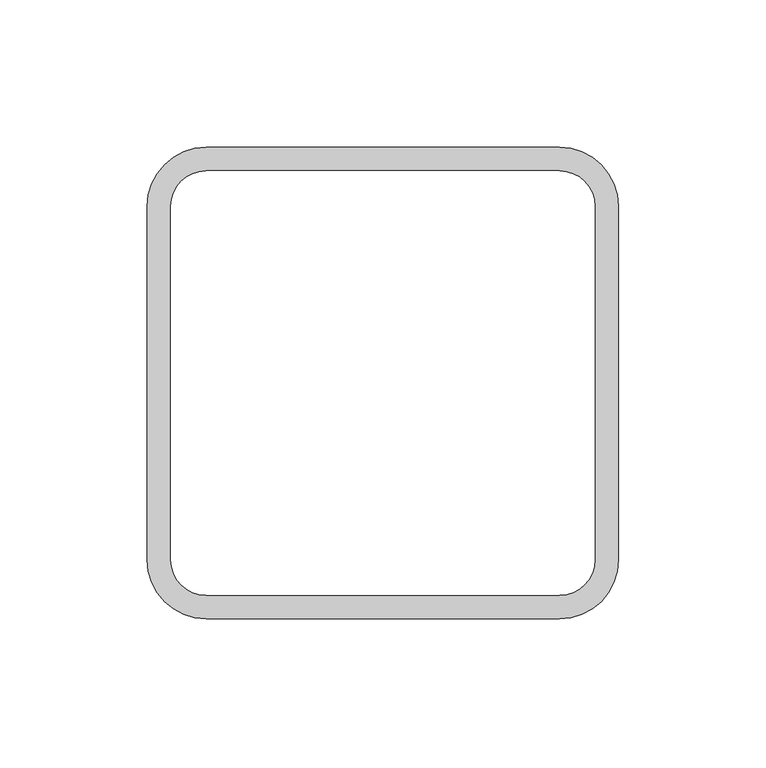
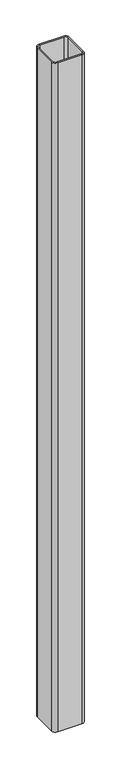
"""IFC4 building model written with IfcOpenShell, lengths in millimetres: column geometry, NLRS_28_SCO_TLB_stalen kolom buisprofiel koudgevormd vierkant-BCPG-MMBS-SRP_gen_rsf : stalen kolom buisprofiel koudgevormd vierkant RHSC_gen__160x160x8."""

from ifc_helpers import new_model, si_unit, point, frame, frame_2d, origin, place, context, project, spatial, polyline, circle_curve, trimmed, segment, composite_curve, outline, extrude, source, transform, mapped, element, save


def column_d8346d76(model_context):
    return source(origin(), model_context, "Body", "SweptSolid", [
        extrude(outline(composite_curve([segment(trimmed(circle_curve(frame_2d((60.0, 60.0)), 20.0), [point((60.0, 80.0))], [point((80.0, 60.0))], False, "CARTESIAN"), True, "CONTINUOUS"), segment(polyline([(80.0, 60.0), (80.0, -60.0)]), True, "CONTINUOUS"), segment(trimmed(circle_curve(frame_2d((60.0, -60.0)), 20.0), [point((80.0, -60.0))], [point((60.0, -80.0))], False, "CARTESIAN"), True, "CONTINUOUS"), segment(polyline([(60.0, -80.0), (-60.0, -80.0)]), True, "CONTINUOUS"), segment(trimmed(circle_curve(frame_2d((-60.0, -60.0)), 20.0), [point((-60.0, -80.0))], [point((-80.0, -60.0))], False, "CARTESIAN"), True, "CONTINUOUS"), segment(polyline([(-80.0, -60.0), (-80.0, 60.0)]), True, "CONTINUOUS"), segment(trimmed(circle_curve(frame_2d((-60.0, 60.0)), 20.0), [point((-80.0, 60.0))], [point((-60.0, 80.0))], False, "CARTESIAN"), True, "CONTINUOUS"), segment(polyline([(-60.0, 80.0), (60.0, 80.0)]), True, "CONTINUOUS")], self_intersect=False), holes=[composite_curve([segment(polyline([(60.0, 72.0), (-60.0, 72.0)]), True, "CONTINUOUS"), segment(trimmed(circle_curve(frame_2d((-60.0, 60.0)), 12.0), [point((-60.0, 72.0))], [point((-72.0, 60.0))], True, "CARTESIAN"), True, "CONTINUOUS"), segment(polyline([(-72.0, 60.0), (-72.0, -60.0)]), True, "CONTINUOUS"), segment(trimmed(circle_curve(frame_2d((-60.0, -60.0)), 12.0), [point((-72.0, -60.0))], [point((-60.0, -72.0))], True, "CARTESIAN"), True, "CONTINUOUS"), segment(polyline([(-60.0, -72.0), (60.0, -72.0)]), True, "CONTINUOUS"), segment(trimmed(circle_curve(frame_2d((60.0, -60.0)), 12.0), [point((60.0, -72.0))], [point((72.0, -60.0))], True, "CARTESIAN"), True, "CONTINUOUS"), segment(polyline([(72.0, -60.0), (72.0, 60.0)]), True, "CONTINUOUS"), segment(trimmed(circle_curve(frame_2d((60.0, 60.0)), 12.0), [point((72.0, 60.0))], [point((60.0, 72.0))], True, "CARTESIAN"), True, "CONTINUOUS")], self_intersect=False)]), frame((0.0, 0.0, -40.0), z_axis=(0.0, 0.0, 1.0), x_axis=(1.0, 0.0, 0.0)), (0.0, 0.0, 1.0), 3510.0),
    ])


if __name__ == "__main__":
    model = new_model("IFC4")
    model_context = context("Model", 3, world=origin())
    ifc_project = project(units=[si_unit("LENGTHUNIT", "METRE", prefix="MILLI")], contexts=[model_context])
    site = spatial("IfcSite", under=ifc_project)
    building = spatial("IfcBuilding", under=site)
    placement = place(None, origin())
    column_shape = column_d8346d76(model_context)
    element("IfcColumn", 1, ObjectType="NLRS_28_SCO_TLB_stalen kolom buisprofiel koudgevormd vierkant-BCPG-MMBS-SRP_gen_rsf : stalen kolom buisprofiel koudgevormd vierkant RHSC_gen__160x160x8", at=placement, inside=building, context=model_context, shape_type="MappedRepresentation", body=[
        mapped(column_shape, transform((0.0, 0.0, 0.0), x_axis=(1.0, 0.0, 0.0), y_axis=(0.0, 1.0, 0.0), z_axis=(0.0, 0.0, 1.0))),
    ])
    save(model, "model.ifc")

# Revit data of these elements
# Type "NLRS_28_SCO_TLB_stalen kolom buisprofiel koudgevormd vierkant-BCPG-MMBS-SRP_gen_rsf : stalen kolom buisprofiel koudgevormd vierkant RHSC_gen__160x160x8"
#   Type IfcGUID = "2$hNzCXOT3YR8V$0Cfyzxk"
#   IfcExportAs = "IfcColumnType"
#   IfcExportType = "COLUMN"
#   Type Comments = "K160x160x8"
#   Model = " "
#   Manufacturer = " "
#   Description = "stalen kolom K160x160x8"
#   Assembly Code = "28.11"
#   vz = 80 mm
#   vy = 80 mm
#   vpz = 80 mm
#   vpy = 80 mm
#   tw = 8 mm
#   tf = 8 mm
#   ri = 20 mm
#   ra = 12 mm
#   d = 160 mm
#   bf = 160 mm
#   NLRS_C_lengte [instance default] = 2743.2 mm
#   Structural Material = NLRS_h2_staal_gen_rsf
#   Keynote = ""
# Element 1 (IfcColumn, "NLRS_28_SCO_TLB_stalen kolom buisprofiel koudgevormd vierkant-BCPG-MMBS-SRP_gen_rsf : stalen kolom buisprofiel koudgevormd vierkant RHSC_gen__160x160x8")
#   NLRS_C_lengte = 3510 mm
#   Materials on its faces: "NLRS_h2_staal_gen_rsf"
# Materials
#   "NLRS_h2_staal_gen_rsf": class "H - Metaal", colour RGB 189 187 185, transparency 0, Keynote = "h2", Manufacturer = "Revit Standards Foundation", URL = "www.revitstandards.org", Description = "staal", Cost = 0
